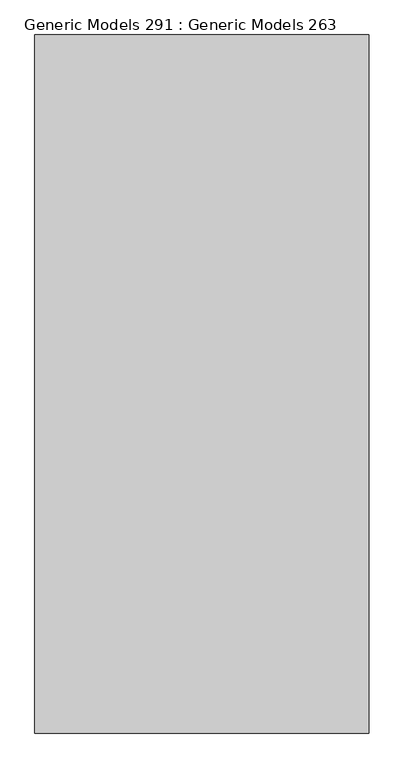
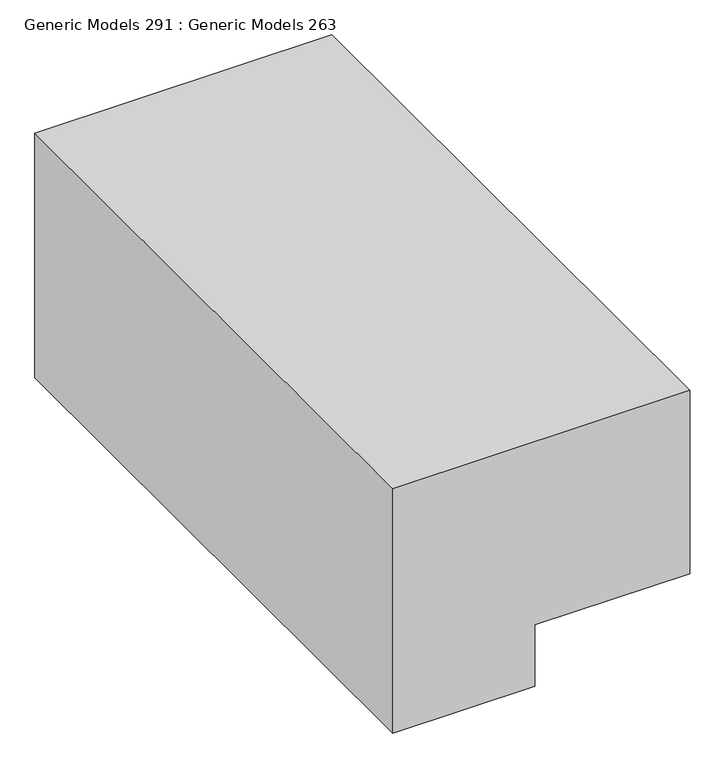
"""IFC4 building model written with IfcOpenShell, lengths in millimetres: proxy geometry, Generic Models 291 : Generic Models 263."""

import ifcopenshell
import ifcopenshell.guid

model = None  # the IFC model being written
_history = None  # IfcOwnerHistory: only IFC2X3 demands one
_inside = {}  # id of a spatial element -> (the spatial element, [elements in it])
_under = {}  # id of a project, library or spatial element -> (it, [spatial elements below it])
_declared = {}  # id of a project -> (the project, [libraries it declares])
_typed = {}  # id of a type object -> (the type object, [elements of that type])
_made_of = {}  # id of a material, layer set ... -> (it, [elements and type objects made of it])


def new_model(schema):
    """Start an empty IFC model of exactly this schema.

    Asked for "IFC4X3", IfcOpenShell would pick the latest addendum, in which some entities
    have other attributes; the version numbers below select the first issue.
    IFC2X3 requires an IfcOwnerHistory on every rooted entity: one is made here for all.
    """
    global model, _history
    if schema == "IFC4X3":
        model = ifcopenshell.file(schema_version=(4, 3, 0, 0))
    else:
        model = ifcopenshell.file(schema=schema)
    _inside.clear()
    _under.clear()
    _declared.clear()
    _typed.clear()
    _made_of.clear()
    _history = None
    if model.schema == "IFC2X3":
        org = make("IfcOrganization", Name="unknown")
        user = make(
            "IfcPersonAndOrganization",
            ThePerson=make("IfcPerson", FamilyName="unknown"),
            TheOrganization=org,
        )
        app = make(
            "IfcApplication",
            ApplicationDeveloper=org,
            Version="unknown",
            ApplicationFullName="unknown",
            ApplicationIdentifier="unknown",
        )
        _history = make(
            "IfcOwnerHistory",
            OwningUser=user,
            OwningApplication=app,
            ChangeAction="ADDED",
            CreationDate=0,
        )
    return model


def make(cls, **values):
    """One entity of the class cls with the attributes given. An attribute that is None is left unset."""
    return model.create_entity(
        cls, **{name: value for name, value in values.items() if value is not None}
    )


def rooted(cls, **values):
    """An entity with a GlobalId (a new one), such as an element, a storey or a relation."""
    return make(cls, GlobalId=ifcopenshell.guid.new(), OwnerHistory=_history, **values)


def si_unit(unit_type, name, prefix=None):
    """IfcSIUnit, for example si_unit("LENGTHUNIT", "METRE", prefix="MILLI")."""
    return make("IfcSIUnit", UnitType=unit_type, Prefix=prefix, Name=name)


def assignment(units):
    """IfcUnitAssignment: the units of a project."""
    return None if units is None else make("IfcUnitAssignment", Units=units)


def point(xyz):
    """IfcCartesianPoint."""
    return None if xyz is None else make("IfcCartesianPoint", Coordinates=xyz)


def direction(xyz):
    """IfcDirection."""
    return None if xyz is None else make("IfcDirection", DirectionRatios=xyz)


def frame(location, z_axis=None, x_axis=None):
    """IfcAxis2Placement3D, a coordinate frame: its origin and axes. An axis left out is left unset."""
    return make(
        "IfcAxis2Placement3D",
        Location=point(location),
        Axis=direction(z_axis),
        RefDirection=direction(x_axis),
    )


def origin():
    """The frame at (0, 0, 0) with its axes left unset."""
    return frame((0.0, 0.0, 0.0))


def place(relative_to, where):
    """IfcLocalPlacement: puts the frame where relative to a parent placement (None: the world)."""
    return make(
        "IfcLocalPlacement", PlacementRelTo=relative_to, RelativePlacement=where
    )


def context(
    kind, dimensions, precision=None, world=None, true_north=None, identifier=None
):
    """IfcGeometricRepresentationContext, for example the 3D "Model" context."""
    return make(
        "IfcGeometricRepresentationContext",
        ContextIdentifier=identifier,
        ContextType=kind,
        CoordinateSpaceDimension=dimensions,
        Precision=precision,
        WorldCoordinateSystem=world,
        TrueNorth=true_north,
    )


def project(units=None, contexts=None):
    """IfcProject with its units and contexts."""
    return rooted(
        "IfcProject",
        Name="project",
        RepresentationContexts=contexts,
        UnitsInContext=assignment(units),
    )


def spatial(cls, under=None, at=None, **own):
    """A site, building, storey or space (cls), placed at a placement, below another one or the project."""
    s = rooted(cls, ObjectPlacement=at, **own)
    if under is not None:
        _under.setdefault(under.id(), (under, []))[1].append(s)
    return s


def polyline(points):
    """IfcPolyline through the points."""
    return make("IfcPolyline", Points=[point(p) for p in points])


def outline(outer, holes=None, kind="AREA"):
    """IfcArbitraryClosedProfileDef: a profile drawn as a closed curve; with holes, ...WithVoids."""
    if holes is None:
        return make("IfcArbitraryClosedProfileDef", ProfileType=kind, OuterCurve=outer)
    return make(
        "IfcArbitraryProfileDefWithVoids",
        ProfileType=kind,
        OuterCurve=outer,
        InnerCurves=holes,
    )


def extrude(swept, where, along, depth):
    """IfcExtrudedAreaSolid: the profile swept, set in the frame where, extruded along a direction by depth."""
    return make(
        "IfcExtrudedAreaSolid",
        SweptArea=swept,
        Position=where,
        ExtrudedDirection=direction(along),
        Depth=depth,
    )


def shape(context_of_items, identifier, shape_type, items):
    """IfcShapeRepresentation: the items that make up one representation, for example the "Body"."""
    return make(
        "IfcShapeRepresentation",
        ContextOfItems=context_of_items,
        RepresentationIdentifier=identifier,
        RepresentationType=shape_type,
        Items=items,
    )


def source(mapping_origin, context_of_items, identifier, shape_type, items):
    """IfcRepresentationMap: a shape defined once, which mapped items show again and again."""
    return make(
        "IfcRepresentationMap",
        MappingOrigin=mapping_origin,
        MappedRepresentation=shape(context_of_items, identifier, shape_type, items),
    )


def transform(
    local_origin,
    x_axis=None,
    y_axis=None,
    z_axis=None,
    scale=None,
    scale2=None,
    scale3=None,
    uniform=True,
):
    """IfcCartesianTransformationOperator3D, or its non-uniform kind. x_axis, y_axis, z_axis: its Axis1, 2, 3."""
    if uniform:
        return make(
            "IfcCartesianTransformationOperator3D",
            Axis1=direction(x_axis),
            Axis2=direction(y_axis),
            LocalOrigin=point(local_origin),
            Scale=scale,
            Axis3=direction(z_axis),
        )
    return make(
        "IfcCartesianTransformationOperator3DnonUniform",
        Axis1=direction(x_axis),
        Axis2=direction(y_axis),
        LocalOrigin=point(local_origin),
        Scale=scale,
        Axis3=direction(z_axis),
        Scale2=scale2,
        Scale3=scale3,
    )


def mapped(mapping_source, mapping_target):
    """IfcMappedItem: shows the shape of a source again, moved by a transform."""
    return make(
        "IfcMappedItem", MappingSource=mapping_source, MappingTarget=mapping_target
    )


def made_of(thing, what):
    """Note that an element or type object is made of a material, layer set ...; save() writes the relation."""
    if what is not None:
        _made_of.setdefault(what.id(), (what, []))[1].append(thing)
    return thing


def element(
    cls,
    number,
    at=None,
    inside=None,
    cuts=None,
    type_object=None,
    material=None,
    context=None,
    identifier="Body",
    shape_type=None,
    held_by="IfcProductDefinitionShape",
    body=None,
    shapes=None,
    **own,
):
    """One element of the class cls, such as IfcWall. Its Tag is "e" and its number.

    at: its placement. inside: the storey or other place that contains it. cuts: it is an
    opening in that element (IfcRelVoidsElement). A single representation is given by context,
    identifier, shape_type and body (its items); several are given by shapes. held_by: the class
    of the entity that holds the representations. save() writes the other relations.
    """
    e = rooted(cls, Tag="e%d" % number, ObjectPlacement=at, **own)
    if body is not None:
        shapes = [shape(context, identifier, shape_type, body)]
    if shapes is not None:
        e.Representation = make(held_by, Representations=shapes)
    if inside is not None:
        _inside.setdefault(inside.id(), (inside, []))[1].append(e)
    if cuts is not None:
        rooted(
            "IfcRelVoidsElement", RelatingBuildingElement=cuts, RelatedOpeningElement=e
        )
    if type_object is not None:
        _typed.setdefault(type_object.id(), (type_object, []))[1].append(e)
    return made_of(e, material)


def aggregate(whole, parts):
    """IfcRelAggregates: a whole, such as a stair, and the parts it consists of."""
    return rooted("IfcRelAggregates", RelatingObject=whole, RelatedObjects=parts)


def save(model, path):
    """Write the relations noted so far, then the file.

    IfcRelAggregates (storeys below a building ...), IfcRelContainedInSpatialStructure (elements
    in a storey), IfcRelDefinesByType, IfcRelAssociatesMaterial and IfcRelDeclares: one each for
    every whole, place, type object, material and project.
    """
    for whole, parts in _under.values():
        aggregate(whole, parts)
    for where, things in _inside.values():
        rooted(
            "IfcRelContainedInSpatialStructure",
            RelatedElements=things,
            RelatingStructure=where,
        )
    for kind, things in _typed.values():
        rooted("IfcRelDefinesByType", RelatedObjects=things, RelatingType=kind)
    for what, things in _made_of.values():
        rooted("IfcRelAssociatesMaterial", RelatedObjects=things, RelatingMaterial=what)
    for by, libraries in _declared.values():
        rooted("IfcRelDeclares", RelatingContext=by, RelatedDefinitions=libraries)
    model.write(path)


def generic_models_291_generic_models_263_452afd1b(model_context):
    return source(origin(), model_context, "Body", "SweptSolid", [
        extrude(outline(polyline([(-381.0, 62319.1797726), (0.0, 62319.1797726), (0.0, 61734.9797726), (-508.0, 61734.9797726), (-508.0, 62014.3797726), (-381.0, 62014.3797726), (-381.0, 62319.1797726)])), frame((0.0, -94.4486541, 0.0), z_axis=(0.0, 1.0, 0.0), x_axis=(0.0, 0.0, 1.0)), (0.0, 0.0, 1.0), 1219.2),
    ])


if __name__ == "__main__":
    model = new_model("IFC4")
    model_context = context("Model", 3, world=origin())
    ifc_project = project(units=[si_unit("LENGTHUNIT", "METRE", prefix="MILLI")], contexts=[model_context])
    site = spatial("IfcSite", under=ifc_project)
    building = spatial("IfcBuilding", under=site)
    placement = place(None, origin())
    generic_models_291_generic_models_263_shape = generic_models_291_generic_models_263_452afd1b(model_context)
    element("IfcBuildingElementProxy", 1, Name="Generic Models 291 : Generic Models 263", ObjectType="Generic Models 291 : Generic Models 263", at=placement, inside=building, context=model_context, shape_type="MappedRepresentation", body=[
        mapped(generic_models_291_generic_models_263_shape, transform((0.0, 0.0, 0.0), x_axis=(1.0, 0.0, 0.0), y_axis=(0.0, 1.0, 0.0), z_axis=(0.0, 0.0, 1.0))),
    ])
    save(model, "model.ifc")

# Revit data of these elements
# Element 1 (IfcBuildingElementProxy, "Generic Models 291 : Generic Models 263")
#   Materials on its faces: "GRADED BACKFILL"
# Materials
#   "GRADED BACKFILL": class "Miscellaneous", colour RGB 128 97 77, transparency 0, Cost = 0
